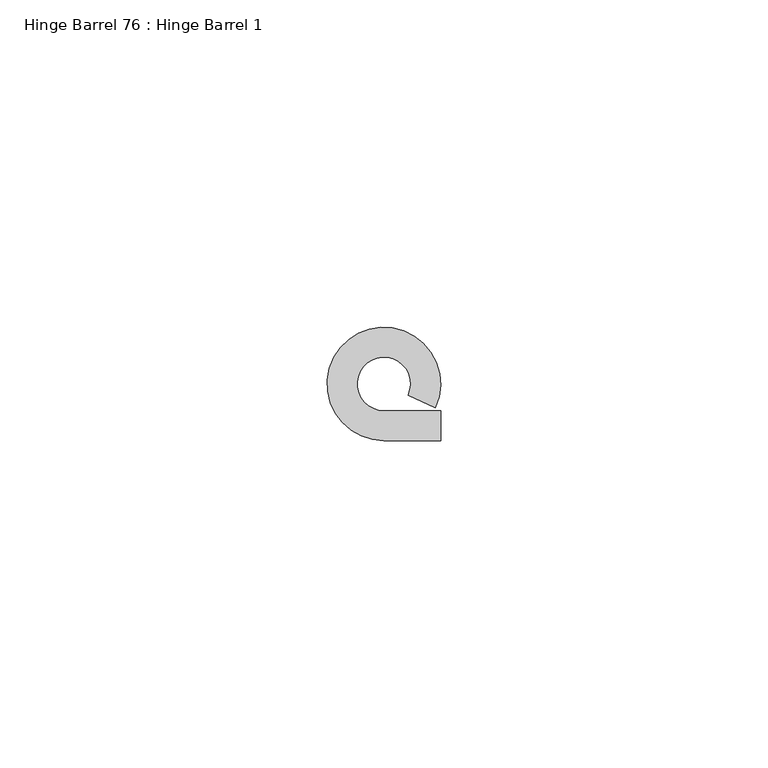
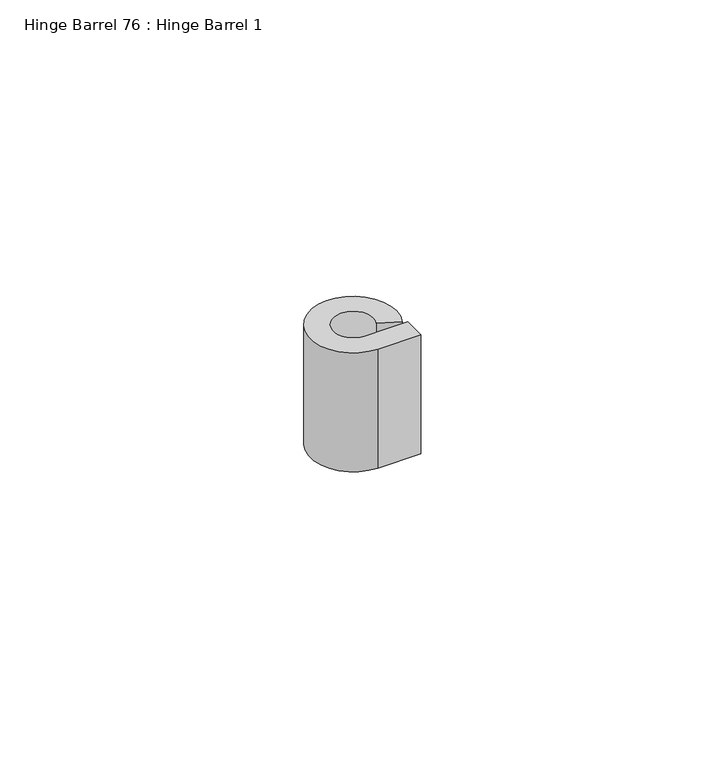
"""IFC4 building model written with IfcOpenShell, lengths in millimetres: proxy geometry, Hinge Barrel 76 : Hinge Barrel 1."""

from ifc_helpers import new_model, si_unit, point, frame, frame_2d, origin, place, context, project, spatial, polyline, circle_curve, trimmed, segment, composite_curve, outline, extrude, source, transform, mapped, element, save


def hinge_barrel_76_hinge_barrel_1_3de8cdcb(model_context):
    return source(origin(), model_context, "Body", "SweptSolid", [
        extrude(outline(composite_curve([segment(polyline([(587323.2214739, -531780.6943841), (587327.7934739, -531780.6943841), (587327.7934739, -531785.2584466), (587319.1320739, -531785.2584466)]), True, "CONTINUOUS"), segment(trimmed(circle_curve(frame_2d((587319.1320739, -531776.6049841)), 8.6534625), [point((587319.1320739, -531785.2584466))], [point((587326.986084, -531780.2377433))], False, "CARTESIAN"), True, "CONTINUOUS"), segment(polyline([(587326.986084, -531780.2377433), (587322.8436736, -531778.321731)]), True, "CONTINUOUS"), segment(trimmed(circle_curve(frame_2d((587319.1320739, -531776.6049841)), 4.0894), [point((587322.8436736, -531778.321731))], [point((587319.1320739, -531780.6943841))], True, "CARTESIAN"), True, "CONTINUOUS"), segment(polyline([(587319.1320739, -531780.6943841), (587323.2214739, -531780.6943841)]), True, "CONTINUOUS")], self_intersect=False)), frame((0.0, 0.0, 412.75), z_axis=(0.0, 0.0, 1.0), x_axis=(1.0, 0.0, 0.0)), (0.0, 0.0, 1.0), 25.4),
    ])


if __name__ == "__main__":
    model = new_model("IFC4")
    model_context = context("Model", 3, world=origin())
    ifc_project = project(units=[si_unit("LENGTHUNIT", "METRE", prefix="MILLI")], contexts=[model_context])
    site = spatial("IfcSite", under=ifc_project)
    building = spatial("IfcBuilding", under=site)
    placement = place(None, origin())
    hinge_barrel_76_hinge_barrel_1_shape = hinge_barrel_76_hinge_barrel_1_3de8cdcb(model_context)
    element("IfcBuildingElementProxy", 1, Name="Hinge Barrel 76 : Hinge Barrel 1", ObjectType="Hinge Barrel 76 : Hinge Barrel 1", at=placement, inside=building, context=model_context, shape_type="MappedRepresentation", body=[
        mapped(hinge_barrel_76_hinge_barrel_1_shape, transform((0.0, 0.0, 0.0), x_axis=(1.0, 0.0, 0.0), y_axis=(0.0, 1.0, 0.0), z_axis=(0.0, 0.0, 1.0))),
    ])
    save(model, "model.ifc")

# Revit data of these elements
# Element 1 (IfcBuildingElementProxy, "Hinge Barrel 76 : Hinge Barrel 1")
#   Materials on its faces: "6\"X6\" WELD-ON STL BUTT HINGE"
# Materials
#   "6\"X6\" WELD-ON STL BUTT HINGE": class "Metal", colour RGB 189 187 185, transparency 0, Description = "Carbon steel", Cost = 0
